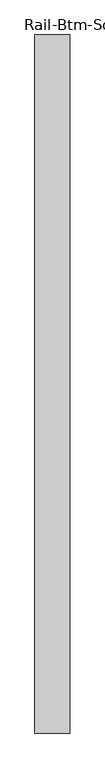
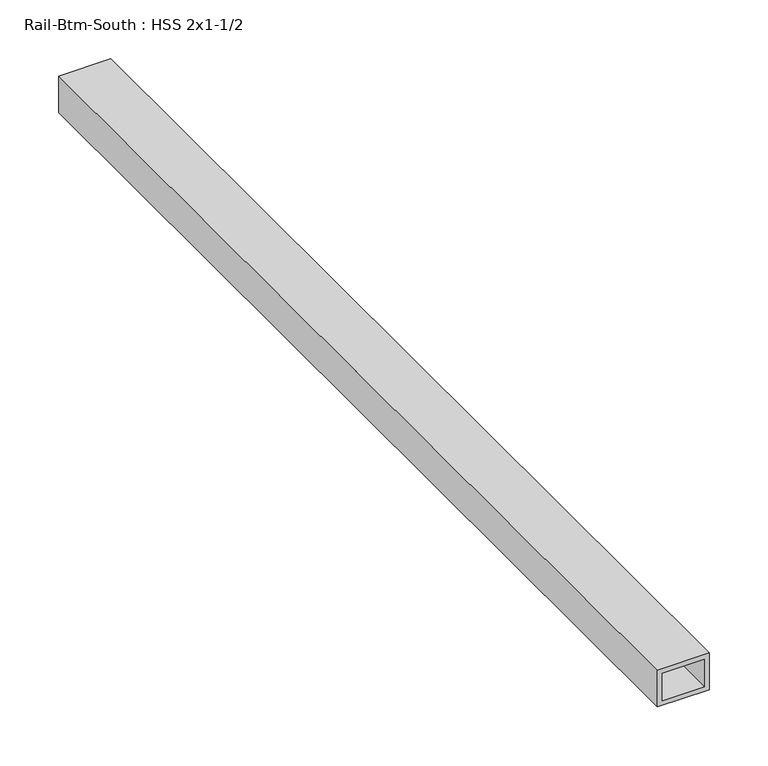
"""IFC4 building model written with IfcOpenShell, lengths in millimetres: proxy geometry, Rail-Btm-South : HSS 2x1-1/2."""

from ifc_helpers import new_model, si_unit, frame, origin, place, context, project, spatial, polyline, outline, extrude, source, transform, mapped, element, save


def rail_btm_south_hss_2x1_1_2_3b7ee801(model_context):
    return source(origin(), model_context, "Body", "SweptSolid", [
        extrude(outline(polyline([(50.8, 587416.6934739), (88.9, 587416.6934739), (88.9, 587365.8934739), (50.8, 587365.8934739), (50.8, 587416.6934739)]), holes=[polyline([(84.1375, 587411.9309739), (55.5625, 587411.9309739), (55.5625, 587370.6559739), (84.1375, 587370.6559739), (84.1375, 587411.9309739)])]), frame((0.0, -533937.9163841, 0.0), z_axis=(0.0, 1.0, 0.0), x_axis=(0.0, 0.0, 1.0)), (0.0, 0.0, 1.0), 1016.0),
    ])


if __name__ == "__main__":
    model = new_model("IFC4")
    model_context = context("Model", 3, world=origin())
    ifc_project = project(units=[si_unit("LENGTHUNIT", "METRE", prefix="MILLI")], contexts=[model_context])
    site = spatial("IfcSite", under=ifc_project)
    building = spatial("IfcBuilding", under=site)
    placement = place(None, origin())
    rail_btm_south_hss_2x1_1_2_shape = rail_btm_south_hss_2x1_1_2_3b7ee801(model_context)
    element("IfcBuildingElementProxy", 1, Name="Rail-Btm-South : HSS 2x1-1/2", ObjectType="Rail-Btm-South : HSS 2x1-1/2", at=placement, inside=building, context=model_context, shape_type="MappedRepresentation", body=[
        mapped(rail_btm_south_hss_2x1_1_2_shape, transform((0.0, 0.0, 0.0), x_axis=(1.0, 0.0, 0.0), y_axis=(0.0, 1.0, 0.0), z_axis=(0.0, 0.0, 1.0))),
    ])
    save(model, "model.ifc")

# Revit data of these elements
# Element 1 (IfcBuildingElementProxy, "Rail-Btm-South : HSS 2x1-1/2")
#   Materials on its faces: "1-1/2\"X2\" GALV. STL HSS TUBING"
# Materials
#   "1-1/2\"X2\" GALV. STL HSS TUBING": class "Generic", colour RGB 211 211 207, transparency 0, Cost = 0
